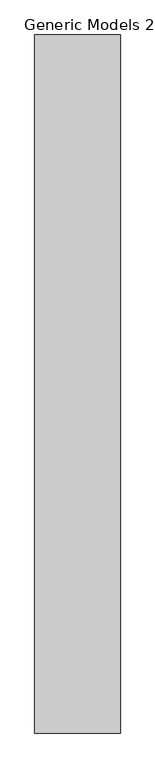
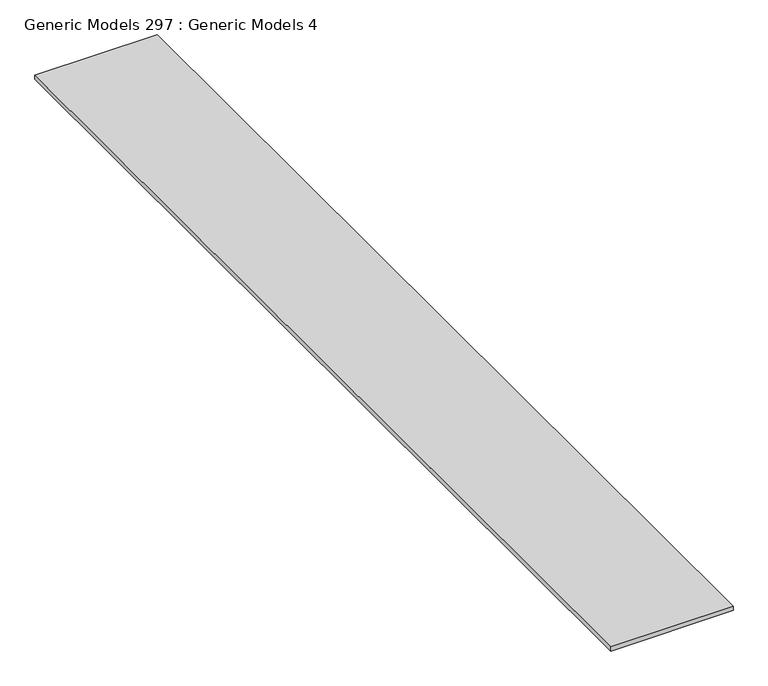
"""IFC4 building model written with IfcOpenShell, lengths in millimetres: proxy geometry, Generic Models 297 : Generic Models 4."""

from ifc_helpers import new_model, si_unit, frame, origin, place, context, project, spatial, polyline, outline, extrude, source, transform, mapped, element, save


def generic_models_297_generic_models_4_16f7774b(model_context):
    return source(origin(), model_context, "Body", "SweptSolid", [
        extrude(outline(polyline([(-5950.1236296, 2583.8769662), (-6498.6122941, 2583.8769662), (-6498.6122941, 7054.2769662), (-5950.1236296, 7054.2769662), (-5950.1236296, 2583.8769662)])), frame((0.0, 0.0, 123278.646), z_axis=(0.0, 0.0, 1.0), x_axis=(1.0, 0.0, 0.0)), (0.0, 0.0, 1.0), 19.05),
    ])


if __name__ == "__main__":
    model = new_model("IFC4")
    model_context = context("Model", 3, world=origin())
    ifc_project = project(units=[si_unit("LENGTHUNIT", "METRE", prefix="MILLI")], contexts=[model_context])
    site = spatial("IfcSite", under=ifc_project)
    building = spatial("IfcBuilding", under=site)
    placement = place(None, origin())
    generic_models_297_generic_models_4_shape = generic_models_297_generic_models_4_16f7774b(model_context)
    element("IfcBuildingElementProxy", 1, Name="Generic Models 297 : Generic Models 4", ObjectType="Generic Models 297 : Generic Models 4", at=placement, inside=building, context=model_context, shape_type="MappedRepresentation", body=[
        mapped(generic_models_297_generic_models_4_shape, transform((0.0, 0.0, 0.0), x_axis=(1.0, 0.0, 0.0), y_axis=(0.0, 1.0, 0.0), z_axis=(0.0, 0.0, 1.0))),
    ])
    save(model, "model.ifc")

# Revit data of these elements
# Element 1 (IfcBuildingElementProxy, "Generic Models 297 : Generic Models 4")
#   Materials on its faces: "_WOOD FLOORING (SPEC T.B.D.)"
# Materials
#   "_WOOD FLOORING (SPEC T.B.D.)": class "Generic", colour RGB 177 130 114, transparency 0, Cost = 0
